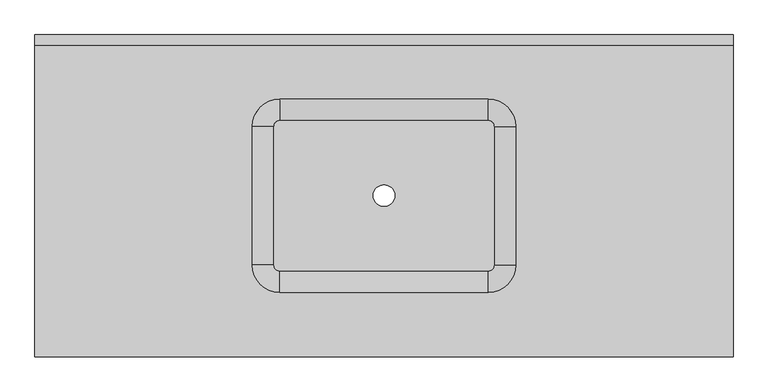
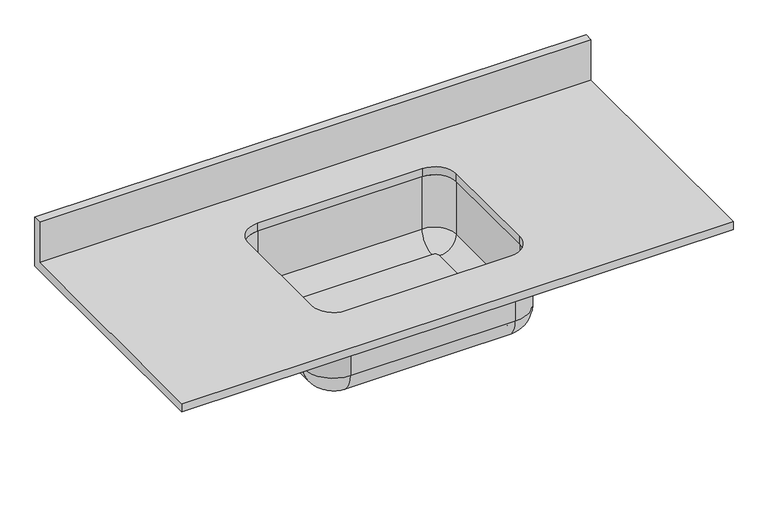
"""IFC4 building model written with IfcOpenShell, lengths in millimetres: furniture geometry, Tampo de Bancada com Cuba : Granilite 60cm."""

from ifc_helpers import new_model, si_unit, point, frame, origin, place, context, project, spatial, polyline, circle_curve, ellipse_curve, trimmed, source, transform, mapped, element, save
from ifc_brep_helpers import plane_surface, cylinder_surface, revolved_surface, advanced_brep


def furniture_832e4139(model_context):
    return source(origin(), model_context, "Body", "AdvancedBrep", [
        advanced_brep(
        [(-356.2622951, -100.0, 880.0), (-744.6622951, -100.0, 880.0), (-815.4622951, -170.8, 880.0), (-815.4622951, -429.2, 880.0), (-744.6622951, -500.0, 880.0), (-356.2622951, -500.0, 880.0), (-285.4622951, -429.2, 880.0), (-285.4622951, -170.8, 880.0), (-356.2622951, -120.0, 880.0), (-305.4622951, -170.8, 880.0), (-305.4622951, -429.2, 880.0), (-356.2622951, -480.0, 880.0), (-744.6622951, -480.0, 880.0), (-795.4622951, -429.2, 880.0), (-795.4622951, -170.8, 880.0), (-744.6622951, -120.0, 880.0), (-356.2622951, -120.0, 750.0), (-305.4622951, -170.8, 750.0), (-305.4622951, -429.2, 750.0), (-356.2622951, -480.0, 750.0), (-744.6622951, -480.0, 750.0), (-795.4622951, -429.2, 750.0), (-795.4622951, -170.8, 750.0), (-744.6622951, -120.0, 750.0), (-356.2622951, -100.0, 750.0), (-744.6622951, -100.0, 750.0), (-815.4622951, -170.8, 750.0), (-815.4622951, -429.2, 750.0), (-744.6622951, -500.0, 750.0), (-356.2622951, -500.0, 750.0), (-285.4622951, -429.2, 750.0), (-285.4622951, -170.8, 750.0), (-345.4622951, -170.8, 710.0), (-356.2622951, -160.0, 710.0), (-744.6622951, -160.0, 710.0), (-755.4622951, -170.8, 710.0), (-755.4622951, -429.2, 710.0), (-744.6622951, -440.0, 710.0), (-356.2622951, -440.0, 710.0), (-345.4622951, -429.2, 710.0), (-570.4622951, -299.5288603, 710.0), (-530.4622951, -299.5288603, 710.0), (-356.2622951, -160.0, 690.0), (-345.4622951, -170.8, 690.0), (-345.4622951, -429.2, 690.0), (-356.2622951, -440.0, 690.0), (-744.6622951, -440.0, 690.0), (-755.4622951, -429.2, 690.0), (-755.4622951, -170.8, 690.0), (-744.6622951, -160.0, 690.0), (-570.4622951, -299.5288603, 690.0), (-530.4622951, -299.5288603, 690.0)],
        [
            (0, 1),
            (1, 2, circle_curve(frame((-744.6622951, -170.8, 880.0), z_axis=(0.0, 0.0, 1.0), x_axis=(1.0, 0.0, 0.0)), 70.8)),
            (2, 3),
            (3, 4, circle_curve(frame((-744.6622951, -429.2, 880.0), z_axis=(0.0, 0.0, 1.0), x_axis=(1.0, 0.0, 0.0)), 70.8)),
            (4, 5),
            (5, 6, circle_curve(frame((-356.2622951, -429.2, 880.0), z_axis=(0.0, 0.0, 1.0), x_axis=(1.0, 0.0, 0.0)), 70.8)),
            (6, 7),
            (7, 0, circle_curve(frame((-356.2622951, -170.8, 880.0), z_axis=(0.0, 0.0, 1.0), x_axis=(1.0, 0.0, 0.0)), 70.8)),
            (8, 9, circle_curve(frame((-356.2622951, -170.8, 880.0), z_axis=(0.0, 0.0, -1.0), x_axis=(1.0, 0.0, 0.0)), 50.8)),
            (9, 10),
            (10, 11, circle_curve(frame((-356.2622951, -429.2, 880.0), z_axis=(0.0, 0.0, -1.0), x_axis=(1.0, 0.0, 0.0)), 50.8)),
            (11, 12),
            (12, 13, circle_curve(frame((-744.6622951, -429.2, 880.0), z_axis=(0.0, 0.0, -1.0), x_axis=(1.0, 0.0, 0.0)), 50.8)),
            (13, 14),
            (14, 15, circle_curve(frame((-744.6622951, -170.8, 880.0), z_axis=(0.0, 0.0, -1.0), x_axis=(1.0, 0.0, 0.0)), 50.8)),
            (15, 8),
            (8, 16),
            (16, 17, circle_curve(frame((-356.2622951, -170.8, 750.0), z_axis=(0.0, 0.0, -1.0), x_axis=(1.0, 0.0, 0.0)), 50.8)),
            (17, 9),
            (17, 18),
            (18, 10),
            (18, 19, circle_curve(frame((-356.2622951, -429.2, 750.0), z_axis=(0.0, 0.0, -1.0), x_axis=(1.0, 0.0, 0.0)), 50.8)),
            (19, 11),
            (19, 20),
            (20, 12),
            (20, 21, circle_curve(frame((-744.6622951, -429.2, 750.0), z_axis=(0.0, 0.0, -1.0), x_axis=(1.0, 0.0, 0.0)), 50.8)),
            (21, 13),
            (21, 22),
            (22, 14),
            (22, 23, circle_curve(frame((-744.6622951, -170.8, 750.0), z_axis=(0.0, 0.0, -1.0), x_axis=(1.0, 0.0, 0.0)), 50.8)),
            (23, 15),
            (23, 16),
            (0, 24),
            (24, 25),
            (25, 1),
            (25, 26, circle_curve(frame((-744.6622951, -170.8, 750.0), z_axis=(0.0, 0.0, 1.0), x_axis=(1.0, 0.0, 0.0)), 70.8)),
            (26, 2),
            (26, 27),
            (27, 3),
            (27, 28, circle_curve(frame((-744.6622951, -429.2, 750.0), z_axis=(0.0, 0.0, 1.0), x_axis=(1.0, 0.0, 0.0)), 70.8)),
            (28, 4),
            (28, 29),
            (29, 5),
            (29, 30, circle_curve(frame((-356.2622951, -429.2, 750.0), z_axis=(0.0, 0.0, 1.0), x_axis=(1.0, 0.0, 0.0)), 70.8)),
            (30, 6),
            (30, 31),
            (31, 7),
            (31, 24, circle_curve(frame((-356.2622951, -170.8, 750.0), z_axis=(0.0, 0.0, 1.0), x_axis=(1.0, 0.0, 0.0)), 70.8)),
            (32, 33, circle_curve(frame((-356.2622951, -170.8, 710.0), z_axis=(0.0, 0.0, 1.0), x_axis=(0.0, 1.0, 0.0)), 10.8)),
            (33, 34),
            (34, 35, circle_curve(frame((-744.6622951, -170.8, 710.0), z_axis=(0.0, 0.0, 1.0), x_axis=(-1.0, 0.0, 0.0)), 10.8)),
            (35, 36),
            (36, 37, circle_curve(frame((-744.6622951, -429.2, 710.0), z_axis=(0.0, 0.0, 1.0), x_axis=(0.0, -1.0, 0.0)), 10.8)),
            (37, 38),
            (38, 39, circle_curve(frame((-356.2622951, -429.2, 710.0), z_axis=(0.0, 0.0, 1.0), x_axis=(1.0, 0.0, 0.0)), 10.8)),
            (39, 32),
            (40, 41, circle_curve(frame((-550.4622951, -299.5288603, 710.0), z_axis=(0.0, 0.0, -1.0), x_axis=(1.0, 0.0, 0.0)), 20.0)),
            (41, 40, circle_curve(frame((-550.4622951, -299.5288603, 710.0), z_axis=(0.0, 0.0, -1.0), x_axis=(1.0, 0.0, 0.0)), 20.0)),
            (42, 43, circle_curve(frame((-356.2622951, -170.8, 690.0), z_axis=(0.0, 0.0, -1.0), x_axis=(0.0, 1.0, 0.0)), 10.8)),
            (43, 44),
            (44, 45, circle_curve(frame((-356.2622951, -429.2, 690.0), z_axis=(0.0, 0.0, -1.0), x_axis=(1.0, 0.0, 0.0)), 10.8)),
            (45, 46),
            (46, 47, circle_curve(frame((-744.6622951, -429.2, 690.0), z_axis=(0.0, 0.0, -1.0), x_axis=(0.0, -1.0, 0.0)), 10.8)),
            (47, 48),
            (48, 49, circle_curve(frame((-744.6622951, -170.8, 690.0), z_axis=(0.0, 0.0, -1.0), x_axis=(-1.0, 0.0, 0.0)), 10.8)),
            (49, 42),
            (50, 51, circle_curve(frame((-550.4622951, -299.5288603, 690.0), z_axis=(0.0, 0.0, 1.0), x_axis=(1.0, 0.0, 0.0)), 20.0)),
            (51, 50, circle_curve(frame((-550.4622951, -299.5288603, 690.0), z_axis=(0.0, 0.0, 1.0), x_axis=(1.0, 0.0, 0.0)), 20.0)),
            (40, 50),
            (51, 41),
            (42, 24, circle_curve(frame((-356.2622951, -160.0, 750.0), z_axis=(1.0, 0.0, 0.0), x_axis=(0.0, 1.0, 0.0)), 60.0)),
            (31, 43, circle_curve(frame((-345.4622951, -170.8, 750.0), z_axis=(0.0, 1.0, 0.0), x_axis=(1.0, 0.0, 0.0)), 60.0)),
            (16, 33, circle_curve(frame((-356.2622951, -160.0, 750.0), z_axis=(-1.0, 0.0, 0.0), x_axis=(0.0, 1.0, 0.0)), 40.0)),
            (32, 17, circle_curve(frame((-345.4622951, -170.8, 750.0), z_axis=(0.0, -1.0, 0.0), x_axis=(1.0, 0.0, 0.0)), 40.0)),
            (30, 44, circle_curve(frame((-345.4622951, -429.2, 750.0), z_axis=(0.0, 1.0, 0.0), x_axis=(1.0, 0.0, 0.0)), 60.0)),
            (39, 18, circle_curve(frame((-345.4622951, -429.2, 750.0), z_axis=(0.0, -1.0, 0.0), x_axis=(1.0, 0.0, 0.0)), 40.0)),
            (29, 45, circle_curve(frame((-356.2622951, -440.0, 750.0), z_axis=(1.0, 0.0, 0.0), x_axis=(0.0, -1.0, 0.0)), 60.0)),
            (38, 19, circle_curve(frame((-356.2622951, -440.0, 750.0), z_axis=(-1.0, 0.0, 0.0), x_axis=(0.0, -1.0, 0.0)), 40.0)),
            (28, 46, circle_curve(frame((-744.6622951, -440.0, 750.0), z_axis=(1.0, 0.0, 0.0), x_axis=(0.0, -1.0, 0.0)), 60.0)),
            (37, 20, circle_curve(frame((-744.6622951, -440.0, 750.0), z_axis=(-1.0, 0.0, 0.0), x_axis=(0.0, -1.0, 0.0)), 40.0)),
            (27, 47, circle_curve(frame((-755.4622951, -429.2, 750.0), z_axis=(0.0, -1.0, 0.0), x_axis=(-1.0, 0.0, 0.0)), 60.0)),
            (36, 21, circle_curve(frame((-755.4622951, -429.2, 750.0), z_axis=(0.0, 1.0, 0.0), x_axis=(-1.0, 0.0, 0.0)), 40.0)),
            (26, 48, circle_curve(frame((-755.4622951, -170.8, 750.0), z_axis=(0.0, -1.0, 0.0), x_axis=(-1.0, 0.0, 0.0)), 60.0)),
            (35, 22, circle_curve(frame((-755.4622951, -170.8, 750.0), z_axis=(0.0, 1.0, 0.0), x_axis=(-1.0, 0.0, 0.0)), 40.0)),
            (25, 49, circle_curve(frame((-744.6622951, -160.0, 750.0), z_axis=(-1.0, 0.0, 0.0), x_axis=(0.0, 1.0, 0.0)), 60.0)),
            (34, 23, circle_curve(frame((-744.6622951, -160.0, 750.0), z_axis=(1.0, 0.0, 0.0), x_axis=(0.0, 1.0, 0.0)), 40.0)),
        ],
        [
            plane_surface(frame((-305.4622951, -170.8, 880.0), z_axis=(0.0, 0.0, 1.0), x_axis=(0.0, -1.0, 0.0))),
            revolved_surface(polyline([(-305.4622951, -170.8, 750.0), (-305.4622951, -170.8, 880.0)]), (-356.2622951, -170.8, 750.0), (0.0, 0.0, -1.0)),
            plane_surface(frame((-305.4622951, -170.8, 880.0), z_axis=(-1.0, 0.0, 0.0), x_axis=(0.0, 0.0, -1.0))),
            revolved_surface(polyline([(-305.4622951, -429.2, 750.0), (-305.4622951, -429.2, 880.0)]), (-356.2622951, -429.2, 750.0), (0.0, 0.0, -1.0)),
            plane_surface(frame((-356.2622951, -480.0, 880.0), z_axis=(0.0, 1.0, 0.0), x_axis=(0.0, 0.0, -1.0))),
            revolved_surface(polyline([(-693.8622951000001, -429.2, 750.0), (-693.8622951000001, -429.2, 880.0)]), (-744.6622951, -429.2, 750.0), (0.0, 0.0, -1.0)),
            plane_surface(frame((-795.4622951, -429.2, 880.0), z_axis=(1.0, 0.0, 0.0), x_axis=(0.0, 0.0, -1.0))),
            revolved_surface(polyline([(-693.8622951000001, -170.8, 750.0), (-693.8622951000001, -170.8, 880.0)]), (-744.6622951, -170.8, 750.0), (0.0, 0.0, -1.0)),
            plane_surface(frame((-744.6622951, -120.0, 880.0), z_axis=(0.0, -1.0, 0.0), x_axis=(0.0, 0.0, -1.0))),
            plane_surface(frame((-356.2622951, -100.0, 880.0), z_axis=(0.0, 1.0, 0.0), x_axis=(0.0, 0.0, -1.0))),
            cylinder_surface(frame((-744.6622951, -170.8, 0.0), z_axis=(0.0, 0.0, 1.0), x_axis=(1.0, 0.0, 0.0)), 70.8),
            plane_surface(frame((-815.4622951, -170.8, 880.0), z_axis=(-1.0, 0.0, 0.0), x_axis=(0.0, 0.0, -1.0))),
            cylinder_surface(frame((-744.6622951, -429.2, 0.0), z_axis=(0.0, 0.0, 1.0), x_axis=(1.0, 0.0, 0.0)), 70.8),
            plane_surface(frame((-744.6622951, -500.0, 880.0), z_axis=(0.0, -1.0, 0.0), x_axis=(0.0, 0.0, -1.0))),
            cylinder_surface(frame((-356.2622951, -429.2, 0.0), z_axis=(0.0, 0.0, 1.0), x_axis=(1.0, 0.0, 0.0)), 70.8),
            plane_surface(frame((-285.4622951, -429.2, 880.0), z_axis=(1.0, 0.0, 0.0), x_axis=(0.0, 0.0, -1.0))),
            cylinder_surface(frame((-356.2622951, -170.8, 0.0), z_axis=(0.0, 0.0, 1.0), x_axis=(1.0, 0.0, 0.0)), 70.8),
            plane_surface(frame((-744.6622951, -160.0, 710.0), z_axis=(0.0, 0.0, 1.0), x_axis=(-1.0, 0.0, 0.0))),
            plane_surface(frame((-744.6622951, -160.0, 690.0), z_axis=(0.0, 0.0, -1.0), x_axis=(1.0, 0.0, 0.0))),
            revolved_surface(polyline([(-530.4622951, -299.5288603, 690.0), (-530.4622951, -299.5288603, 710.0)]), (-550.4622951, -299.5288603, 0.0), (0.0, 0.0, -1.0)),
            revolved_surface(trimmed(ellipse_curve(frame((-356.2622951, -160.0, 750.0), z_axis=(-1.0, 0.0, 0.0), x_axis=(0.0, 1.0, 0.0)), 60.0, 60.0), [point((-356.2622951, -100.0, 750.0))], [point((-356.2622951, -160.0, 690.0))], True, "CARTESIAN"), (-356.2622951, -170.8, 0.0), (0.0, 0.0, -1.0)),
            revolved_surface(trimmed(ellipse_curve(frame((-356.2622951, -160.0, 750.0), z_axis=(1.0, 0.0, 0.0), x_axis=(0.0, 1.0, 0.0)), 40.0, 40.0), [point((-356.2622951, -160.0, 710.0))], [point((-356.2622951, -120.0, 750.0))], True, "CARTESIAN"), (-356.2622951, -170.8, 0.0), (0.0, 0.0, -1.0)),
            cylinder_surface(frame((-345.4622951, -170.8, 750.0), z_axis=(0.0, 1.0, 0.0), x_axis=(1.0, 0.0, 0.0)), 60.0),
            revolved_surface(polyline([(-305.4622951, -429.2, 750.0), (-305.4622951, -170.8, 750.0)]), (-345.4622951, -170.8, 750.0), (0.0, -1.0, 0.0)),
            revolved_surface(trimmed(ellipse_curve(frame((-345.4622951, -429.2, 750.0), z_axis=(0.0, 1.0, 0.0), x_axis=(1.0, 0.0, 0.0)), 60.0, 60.0), [point((-285.4622951, -429.2, 750.0))], [point((-345.4622951, -429.2, 690.0))], True, "CARTESIAN"), (-356.2622951, -429.2, 0.0), (0.0, 0.0, -1.0)),
            revolved_surface(trimmed(ellipse_curve(frame((-345.4622951, -429.2, 750.0), z_axis=(0.0, -1.0, 0.0), x_axis=(1.0, 0.0, 0.0)), 40.0, 40.0), [point((-345.4622951, -429.2, 710.0))], [point((-305.4622951, -429.2, 750.0))], True, "CARTESIAN"), (-356.2622951, -429.2, 0.0), (0.0, 0.0, -1.0)),
            cylinder_surface(frame((-356.2622951, -440.0, 750.0), z_axis=(1.0, 0.0, 0.0), x_axis=(0.0, -1.0, 0.0)), 60.0),
            revolved_surface(polyline([(-744.6622951, -480.0, 750.0), (-356.2622951, -480.0, 750.0)]), (-356.2622951, -440.0, 750.0), (-1.0, 0.0, 0.0)),
            revolved_surface(trimmed(ellipse_curve(frame((-744.6622951, -440.0, 750.0), z_axis=(1.0, 0.0, 0.0), x_axis=(0.0, -1.0, 0.0)), 60.0, 60.0), [point((-744.6622951, -500.0, 750.0))], [point((-744.6622951, -440.0, 690.0))], True, "CARTESIAN"), (-744.6622951, -429.2, 0.0), (0.0, 0.0, -1.0)),
            revolved_surface(trimmed(ellipse_curve(frame((-744.6622951, -440.0, 750.0), z_axis=(-1.0, 0.0, 0.0), x_axis=(0.0, -1.0, 0.0)), 40.0, 40.0), [point((-744.6622951, -440.0, 710.0))], [point((-744.6622951, -480.0, 750.0))], True, "CARTESIAN"), (-744.6622951, -429.2, 0.0), (0.0, 0.0, -1.0)),
            cylinder_surface(frame((-755.4622951, -429.2, 750.0), z_axis=(0.0, -1.0, 0.0), x_axis=(-1.0, 0.0, 0.0)), 60.0),
            revolved_surface(polyline([(-795.4622951, -170.8, 750.0), (-795.4622951, -429.2, 750.0)]), (-755.4622951, -429.2, 750.0), (0.0, 1.0, 0.0)),
            revolved_surface(trimmed(ellipse_curve(frame((-755.4622951, -170.8, 750.0), z_axis=(0.0, -1.0, 0.0), x_axis=(-1.0, 0.0, 0.0)), 60.0, 60.0), [point((-815.4622951, -170.8, 750.0))], [point((-755.4622951, -170.8, 690.0))], True, "CARTESIAN"), (-744.6622951, -170.8, 0.0), (0.0, 0.0, -1.0)),
            revolved_surface(trimmed(ellipse_curve(frame((-755.4622951, -170.8, 750.0), z_axis=(0.0, 1.0, 0.0), x_axis=(-1.0, 0.0, 0.0)), 40.0, 40.0), [point((-755.4622951, -170.8, 710.0))], [point((-795.4622951, -170.8, 750.0))], True, "CARTESIAN"), (-744.6622951, -170.8, 0.0), (0.0, 0.0, -1.0)),
            cylinder_surface(frame((-744.6622951, -160.0, 750.0), z_axis=(-1.0, 0.0, 0.0), x_axis=(0.0, 1.0, 0.0)), 60.0),
            revolved_surface(polyline([(-356.2622951, -120.0, 750.0), (-744.6622951, -120.0, 750.0)]), (-744.6622951, -160.0, 750.0), (1.0, 0.0, 0.0)),
        ],
        [
            (0, [[1, 2, 3, 4, 5, 6, 7, 8], [9, 10, 11, 12, 13, 14, 15, 16]]),
            (1, [[-9, 17, 18, 19]]),
            (2, [[-10, -19, 20, 21]]),
            (3, [[-11, -21, 22, 23]]),
            (4, [[-12, -23, 24, 25]]),
            (5, [[-13, -25, 26, 27]]),
            (6, [[-14, -27, 28, 29]]),
            (7, [[-15, -29, 30, 31]]),
            (8, [[-16, -31, 32, -17]]),
            (9, [[-1, 33, 34, 35]]),
            (10, [[-2, -35, 36, 37]]),
            (11, [[-3, -37, 38, 39]]),
            (12, [[-4, -39, 40, 41]]),
            (13, [[-5, -41, 42, 43]]),
            (14, [[-6, -43, 44, 45]]),
            (15, [[-7, -45, 46, 47]]),
            (16, [[-8, -47, 48, -33]]),
            (17, [[49, 50, 51, 52, 53, 54, 55, 56], [57, 58]]),
            (18, [[59, 60, 61, 62, 63, 64, 65, 66], [67, 68]]),
            (19, [[-57, 69, -68, 70]]),
            (19, [[-58, -70, -67, -69]]),
            (20, [[71, -48, 72, -59]]),
            (21, [[73, -49, 74, -18]]),
            (22, [[-72, -46, 75, -60]]),
            (23, [[-74, -56, 76, -20]]),
            (24, [[-75, -44, 77, -61]]),
            (25, [[-76, -55, 78, -22]]),
            (26, [[-77, -42, 79, -62]]),
            (27, [[-78, -54, 80, -24]]),
            (28, [[-79, -40, 81, -63]]),
            (29, [[-80, -53, 82, -26]]),
            (30, [[-81, -38, 83, -64]]),
            (31, [[-82, -52, 84, -28]]),
            (32, [[-83, -36, 85, -65]]),
            (33, [[-84, -51, 86, -30]]),
            (34, [[-71, -66, -85, -34]]),
            (35, [[-73, -32, -86, -50]]),
        ],
    ),
        advanced_brep(
        [(-1200.4622951, -600.0, 900.0), (99.5377049, -600.0, 900.0), (99.5377049, -19.05, 900.0), (-1200.4622951, -19.05, 900.0), (-744.6622951, -120.0, 900.0), (-356.2622951, -120.0, 900.0), (-305.4622951, -170.8, 900.0), (-305.4622951, -429.2, 900.0), (-356.2622951, -480.0, 900.0), (-744.6622951, -480.0, 900.0), (-795.4622951, -429.2, 900.0), (-795.4622951, -170.8, 900.0), (99.5377049, 0.0, 880.0), (99.5377049, -600.0, 880.0), (-1200.4622951, -600.0, 880.0), (-1200.4622951, 0.0, 880.0), (-356.2622951, -120.0, 880.0), (-744.6622951, -120.0, 880.0), (-795.4622951, -170.8, 880.0), (-795.4622951, -429.2, 880.0), (-744.6622951, -480.0, 880.0), (-356.2622951, -480.0, 880.0), (-305.4622951, -429.2, 880.0), (-305.4622951, -170.8, 880.0), (-1200.4622951, 0.0, 1001.6), (99.5377049, 0.0, 1001.6), (-1200.4622951, -19.05, 1001.6), (99.5377049, -19.05, 1001.6)],
        [
            (0, 1),
            (1, 2),
            (2, 3),
            (3, 0),
            (4, 5),
            (5, 6, circle_curve(frame((-356.2622951, -170.8, 900.0), z_axis=(0.0, 0.0, -1.0), x_axis=(1.0, 0.0, 0.0)), 50.8)),
            (6, 7),
            (7, 8, circle_curve(frame((-356.2622951, -429.2, 900.0), z_axis=(0.0, 0.0, -1.0), x_axis=(1.0, 0.0, 0.0)), 50.8)),
            (8, 9),
            (9, 10, circle_curve(frame((-744.6622951, -429.2, 900.0), z_axis=(0.0, 0.0, -1.0), x_axis=(1.0, 0.0, 0.0)), 50.8)),
            (10, 11),
            (11, 4, circle_curve(frame((-744.6622951, -170.8, 900.0), z_axis=(0.0, 0.0, -1.0), x_axis=(1.0, 0.0, 0.0)), 50.8)),
            (12, 13),
            (13, 14),
            (14, 15),
            (15, 12),
            (16, 17),
            (17, 18, circle_curve(frame((-744.6622951, -170.8, 880.0), z_axis=(0.0, 0.0, 1.0), x_axis=(1.0, 0.0, 0.0)), 50.8)),
            (18, 19),
            (19, 20, circle_curve(frame((-744.6622951, -429.2, 880.0), z_axis=(0.0, 0.0, 1.0), x_axis=(1.0, 0.0, 0.0)), 50.8)),
            (20, 21),
            (21, 22, circle_curve(frame((-356.2622951, -429.2, 880.0), z_axis=(0.0, 0.0, 1.0), x_axis=(1.0, 0.0, 0.0)), 50.8)),
            (22, 23),
            (23, 16, circle_curve(frame((-356.2622951, -170.8, 880.0), z_axis=(0.0, 0.0, 1.0), x_axis=(1.0, 0.0, 0.0)), 50.8)),
            (15, 24),
            (24, 25),
            (25, 12),
            (14, 0),
            (3, 26),
            (26, 24),
            (13, 1),
            (25, 27),
            (27, 2),
            (26, 27),
            (4, 17),
            (16, 5),
            (11, 18),
            (10, 19),
            (9, 20),
            (8, 21),
            (7, 22),
            (6, 23),
        ],
        [
            plane_surface(frame((-1200.4622951, 0.0, 900.0), z_axis=(0.0, 0.0, 1.0), x_axis=(-1.0, 0.0, 0.0))),
            plane_surface(frame((-1200.4622951, 0.0, 880.0), z_axis=(0.0, 0.0, -1.0), x_axis=(1.0, 0.0, 0.0))),
            plane_surface(frame((99.5377049, 0.0, 900.0), z_axis=(0.0, 1.0, 0.0), x_axis=(0.0, 0.0, -1.0))),
            plane_surface(frame((-1200.4622951, 0.0, 900.0), z_axis=(-1.0, 0.0, 0.0), x_axis=(0.0, 0.0, -1.0))),
            plane_surface(frame((-1200.4622951, -600.0, 900.0), z_axis=(0.0, -1.0, 0.0), x_axis=(0.0, 0.0, -1.0))),
            plane_surface(frame((99.5377049, -600.0, 900.0), z_axis=(1.0, 0.0, 0.0), x_axis=(0.0, 0.0, -1.0))),
            plane_surface(frame((-1200.4622951, 0.0, 1001.6), z_axis=(0.0, 0.0, 1.0), x_axis=(0.0, -1.0, 0.0))),
            plane_surface(frame((-1200.4622951, -19.05, 1001.6), z_axis=(0.0, -1.0, 0.0), x_axis=(0.0, 0.0, -1.0))),
            plane_surface(frame((-356.2622951, -120.0, 900.0), z_axis=(0.0, -1.0, 0.0), x_axis=(0.0, 0.0, -1.0))),
            revolved_surface(polyline([(-693.8622951000001, -170.8, 900.0), (-693.8622951000001, -170.8, 880.0)]), (-744.6622951, -170.8, 880.0), (0.0, 0.0, 1.0)),
            plane_surface(frame((-795.4622951, -170.8, 900.0), z_axis=(1.0, 0.0, 0.0), x_axis=(0.0, 0.0, -1.0))),
            revolved_surface(polyline([(-693.8622951000001, -429.2, 900.0), (-693.8622951000001, -429.2, 880.0)]), (-744.6622951, -429.2, 880.0), (0.0, 0.0, 1.0)),
            plane_surface(frame((-744.6622951, -480.0, 900.0), z_axis=(0.0, 1.0, 0.0), x_axis=(0.0, 0.0, -1.0))),
            revolved_surface(polyline([(-305.4622951, -429.2, 900.0), (-305.4622951, -429.2, 880.0)]), (-356.2622951, -429.2, 880.0), (0.0, 0.0, 1.0)),
            plane_surface(frame((-305.4622951, -429.2, 900.0), z_axis=(-1.0, 0.0, 0.0), x_axis=(0.0, 0.0, -1.0))),
            revolved_surface(polyline([(-305.4622951, -170.8, 900.0), (-305.4622951, -170.8, 880.0)]), (-356.2622951, -170.8, 880.0), (0.0, 0.0, 1.0)),
        ],
        [
            (0, [[1, 2, 3, 4], [5, 6, 7, 8, 9, 10, 11, 12]]),
            (1, [[13, 14, 15, 16], [17, 18, 19, 20, 21, 22, 23, 24]]),
            (2, [[-16, 25, 26, 27]]),
            (3, [[-15, 28, -4, 29, 30, -25]]),
            (4, [[-1, -28, -14, 31]]),
            (5, [[-13, -27, 32, 33, -2, -31]]),
            (6, [[-30, 34, -32, -26]]),
            (7, [[-34, -29, -3, -33]]),
            (8, [[35, -17, 36, -5]]),
            (9, [[-35, -12, 37, -18]]),
            (10, [[-37, -11, 38, -19]]),
            (11, [[-38, -10, 39, -20]]),
            (12, [[-39, -9, 40, -21]]),
            (13, [[-40, -8, 41, -22]]),
            (14, [[-41, -7, 42, -23]]),
            (15, [[-36, -24, -42, -6]]),
        ],
    ),
    ])


if __name__ == "__main__":
    model = new_model("IFC4")
    model_context = context("Model", 3, world=origin())
    ifc_project = project(units=[si_unit("LENGTHUNIT", "METRE", prefix="MILLI")], contexts=[model_context])
    site = spatial("IfcSite", under=ifc_project)
    building = spatial("IfcBuilding", under=site)
    placement = place(None, origin())
    furniture_shape = furniture_832e4139(model_context)
    element("IfcFurniture", 1, ObjectType="Tampo de Bancada com Cuba : Granilite 60cm", at=placement, inside=building, context=model_context, shape_type="MappedRepresentation", body=[
        mapped(furniture_shape, transform((0.0, 0.0, 0.0), x_axis=(1.0, 0.0, 0.0), y_axis=(0.0, 1.0, 0.0), z_axis=(0.0, 0.0, 1.0))),
    ])
    save(model, "model.ifc")

# Revit data of these elements
# Type "Tampo de Bancada com Cuba : Granilite 60cm"
#   SINAPI = ""
#   Espessura da bancada = 2.00 cm
#   Depth = 60.00 cm
#   Altura da Cuba = 19.00 cm
#   Height = 90.00 cm
#   Comprimento [instance default] = 120.00 cm
#   Localização da pia [instance default] = 60.00 cm
#   Localização da pia em relação a parede [instance default] = 12.00 cm
#   Profundidade de abertura da pia [instance default] = 36.00 cm
#   Largura da abertura da pia [instance default] = 49.00 cm
#   Material do topo da bancada = Granilite Sintético
#   Assembly Code = ""
# Element 1 (IfcFurniture, "Tampo de Bancada com Cuba : Granilite 60cm")
#   Comprimento = 130.00 cm
#   Localização da pia = 65.00 cm
#   Materials on its faces: "Granilite Sintético"
# Materials
#   "Granilite Sintético": class "Resina", colour RGB 81 80 80, transparency 0, Cost = 0
